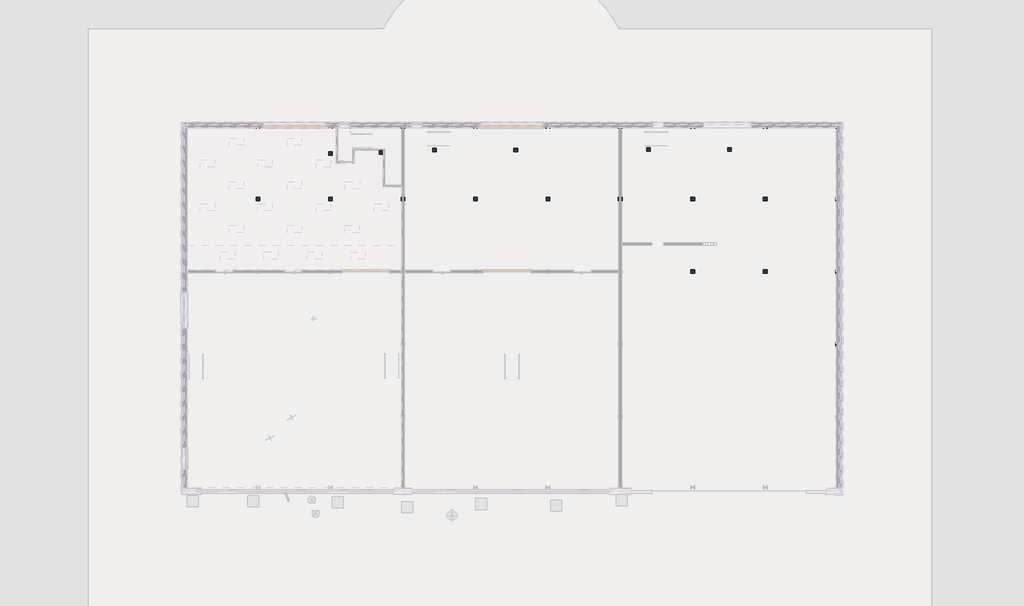
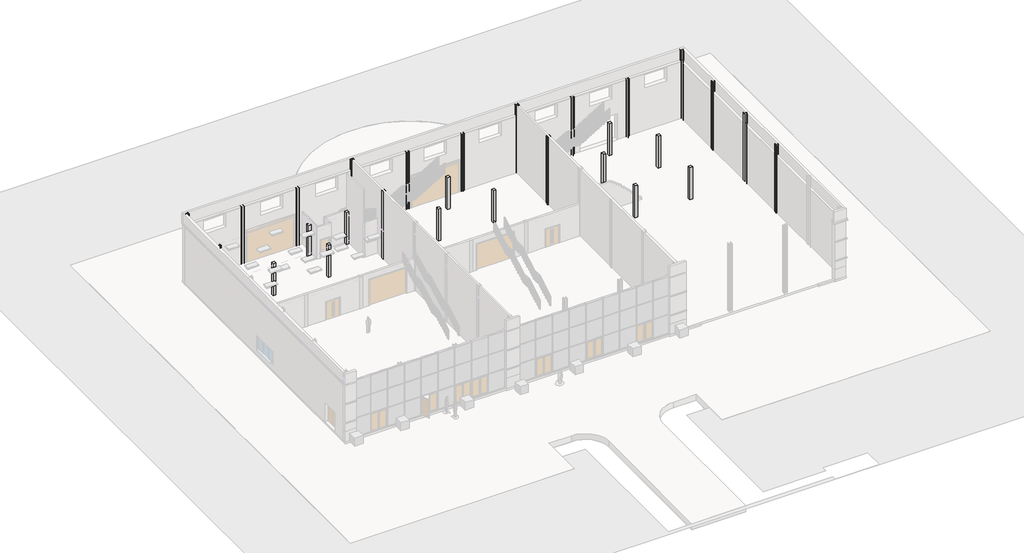
# One storey, part 6 of 13: 30 columns, 25 slabs, 2 footings.
# Revit data of these elements (continued)
# Elements 15, 16, 17, 18, 19, 20, 21, 22, 23, 24, 25, 26, 27, 28, 29, 30 (IfcColumn, "UC-Universal Column-Column : 305x305x97UC")
#   Comments = ""
#   Structural Material = Steel, 45-345
#   Phase Created = New Construction
#   Materials on its faces: "Steel, 45-345"
# Elements 31, 32 (IfcFooting, "Wall Foundation - Commercial 1300 x 450")
#   Phase Created = New Construction
#   Materials on its faces: "Concrete, Cast In Situ"
# Elements 33, 34, 35, 36, 37, 38, 39, 40, 41, 42, 43, 44, 45, 46, 47, 48, 49, 50, 51, 52, 53, 54, 55, 56, 57 (IfcSlab, "Pad Foundation-Rectangular : 1000x1000x500")
#   Comments = ""
#   Reinforcement Specs = ""
#   Mesh = ""
#   Concrete Grade = ""
#   Structural Material = Concrete - Cast-in-Place Concrete
#   Phase Created = New Construction
#   Materials on its faces: "Concrete - Cast-in-Place Concrete"
# Materials
#   "Concrete - Cast-in-Place Concrete": class "Concrete", colour RGB 192 192 192, transparency 0
#   "Steel, 45-345": class "Metal", colour RGB 247 247 247, transparency 0, Description = "Steel 345 MPa", Cost = 0
#   "Concrete, Cast In Situ": class "Concrete", colour RGB 192 192 192, transparency 0, Description = "physical material", Cost = 0
